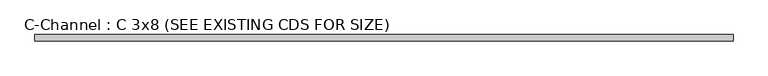
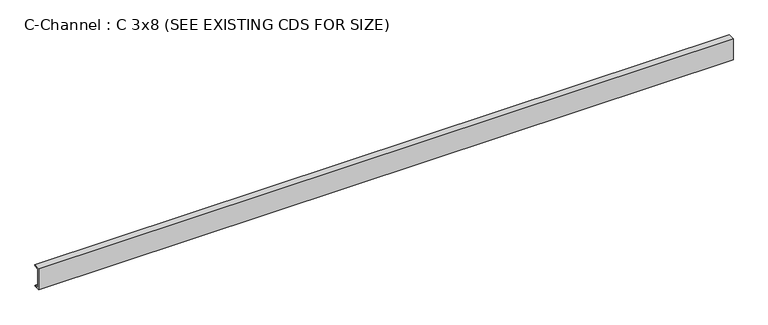
"""IFC4 building model written with IfcOpenShell, lengths in millimetres: beam geometry, C-Channel : C 3x8 (SEE EXISTING CDS FOR SIZE)."""

import ifcopenshell
import ifcopenshell.guid

model = None  # the IFC model being written
_history = None  # IfcOwnerHistory: only IFC2X3 demands one
_inside = {}  # id of a spatial element -> (the spatial element, [elements in it])
_under = {}  # id of a project, library or spatial element -> (it, [spatial elements below it])
_declared = {}  # id of a project -> (the project, [libraries it declares])
_typed = {}  # id of a type object -> (the type object, [elements of that type])
_made_of = {}  # id of a material, layer set ... -> (it, [elements and type objects made of it])


def new_model(schema):
    """Start an empty IFC model of exactly this schema.

    Asked for "IFC4X3", IfcOpenShell would pick the latest addendum, in which some entities
    have other attributes; the version numbers below select the first issue.
    IFC2X3 requires an IfcOwnerHistory on every rooted entity: one is made here for all.
    """
    global model, _history
    if schema == "IFC4X3":
        model = ifcopenshell.file(schema_version=(4, 3, 0, 0))
    else:
        model = ifcopenshell.file(schema=schema)
    _inside.clear()
    _under.clear()
    _declared.clear()
    _typed.clear()
    _made_of.clear()
    _history = None
    if model.schema == "IFC2X3":
        org = make("IfcOrganization", Name="unknown")
        user = make(
            "IfcPersonAndOrganization",
            ThePerson=make("IfcPerson", FamilyName="unknown"),
            TheOrganization=org,
        )
        app = make(
            "IfcApplication",
            ApplicationDeveloper=org,
            Version="unknown",
            ApplicationFullName="unknown",
            ApplicationIdentifier="unknown",
        )
        _history = make(
            "IfcOwnerHistory",
            OwningUser=user,
            OwningApplication=app,
            ChangeAction="ADDED",
            CreationDate=0,
        )
    return model


def make(cls, **values):
    """One entity of the class cls with the attributes given. An attribute that is None is left unset."""
    return model.create_entity(
        cls, **{name: value for name, value in values.items() if value is not None}
    )


def rooted(cls, **values):
    """An entity with a GlobalId (a new one), such as an element, a storey or a relation."""
    return make(cls, GlobalId=ifcopenshell.guid.new(), OwnerHistory=_history, **values)


def si_unit(unit_type, name, prefix=None):
    """IfcSIUnit, for example si_unit("LENGTHUNIT", "METRE", prefix="MILLI")."""
    return make("IfcSIUnit", UnitType=unit_type, Prefix=prefix, Name=name)


def assignment(units):
    """IfcUnitAssignment: the units of a project."""
    return None if units is None else make("IfcUnitAssignment", Units=units)


def point(xyz):
    """IfcCartesianPoint."""
    return None if xyz is None else make("IfcCartesianPoint", Coordinates=xyz)


def direction(xyz):
    """IfcDirection."""
    return None if xyz is None else make("IfcDirection", DirectionRatios=xyz)


def frame(location, z_axis=None, x_axis=None):
    """IfcAxis2Placement3D, a coordinate frame: its origin and axes. An axis left out is left unset."""
    return make(
        "IfcAxis2Placement3D",
        Location=point(location),
        Axis=direction(z_axis),
        RefDirection=direction(x_axis),
    )


def frame_2d(location, x_axis=None):
    """IfcAxis2Placement2D, a coordinate frame in the plane: its origin and x axis."""
    return make(
        "IfcAxis2Placement2D", Location=point(location), RefDirection=direction(x_axis)
    )


def origin():
    """The frame at (0, 0, 0) with its axes left unset."""
    return frame((0.0, 0.0, 0.0))


def place(relative_to, where):
    """IfcLocalPlacement: puts the frame where relative to a parent placement (None: the world)."""
    return make(
        "IfcLocalPlacement", PlacementRelTo=relative_to, RelativePlacement=where
    )


def context(
    kind, dimensions, precision=None, world=None, true_north=None, identifier=None
):
    """IfcGeometricRepresentationContext, for example the 3D "Model" context."""
    return make(
        "IfcGeometricRepresentationContext",
        ContextIdentifier=identifier,
        ContextType=kind,
        CoordinateSpaceDimension=dimensions,
        Precision=precision,
        WorldCoordinateSystem=world,
        TrueNorth=true_north,
    )


def project(units=None, contexts=None):
    """IfcProject with its units and contexts."""
    return rooted(
        "IfcProject",
        Name="project",
        RepresentationContexts=contexts,
        UnitsInContext=assignment(units),
    )


def spatial(cls, under=None, at=None, **own):
    """A site, building, storey or space (cls), placed at a placement, below another one or the project."""
    s = rooted(cls, ObjectPlacement=at, **own)
    if under is not None:
        _under.setdefault(under.id(), (under, []))[1].append(s)
    return s


def polyline(points):
    """IfcPolyline through the points."""
    return make("IfcPolyline", Points=[point(p) for p in points])


def circle_curve(where, radius):
    """IfcCircle in the frame where."""
    return make("IfcCircle", Position=where, Radius=radius)


def trimmed(basis, trim1, trim2, sense, master):
    """IfcTrimmedCurve: the piece of a basis curve between two trims."""
    return make(
        "IfcTrimmedCurve",
        BasisCurve=basis,
        Trim1=trim1,
        Trim2=trim2,
        SenseAgreement=sense,
        MasterRepresentation=master,
    )


def segment(curve, same_sense, transition):
    """IfcCompositeCurveSegment."""
    return make(
        "IfcCompositeCurveSegment",
        Transition=transition,
        SameSense=same_sense,
        ParentCurve=curve,
    )


def composite_curve(segments, self_intersect=None):
    """IfcCompositeCurve: segments joined end to end."""
    return make("IfcCompositeCurve", Segments=segments, SelfIntersect=self_intersect)


def outline(outer, holes=None, kind="AREA"):
    """IfcArbitraryClosedProfileDef: a profile drawn as a closed curve; with holes, ...WithVoids."""
    if holes is None:
        return make("IfcArbitraryClosedProfileDef", ProfileType=kind, OuterCurve=outer)
    return make(
        "IfcArbitraryProfileDefWithVoids",
        ProfileType=kind,
        OuterCurve=outer,
        InnerCurves=holes,
    )


def extrude(swept, where, along, depth):
    """IfcExtrudedAreaSolid: the profile swept, set in the frame where, extruded along a direction by depth."""
    return make(
        "IfcExtrudedAreaSolid",
        SweptArea=swept,
        Position=where,
        ExtrudedDirection=direction(along),
        Depth=depth,
    )


def shape(context_of_items, identifier, shape_type, items):
    """IfcShapeRepresentation: the items that make up one representation, for example the "Body"."""
    return make(
        "IfcShapeRepresentation",
        ContextOfItems=context_of_items,
        RepresentationIdentifier=identifier,
        RepresentationType=shape_type,
        Items=items,
    )


def source(mapping_origin, context_of_items, identifier, shape_type, items):
    """IfcRepresentationMap: a shape defined once, which mapped items show again and again."""
    return make(
        "IfcRepresentationMap",
        MappingOrigin=mapping_origin,
        MappedRepresentation=shape(context_of_items, identifier, shape_type, items),
    )


def transform(
    local_origin,
    x_axis=None,
    y_axis=None,
    z_axis=None,
    scale=None,
    scale2=None,
    scale3=None,
    uniform=True,
):
    """IfcCartesianTransformationOperator3D, or its non-uniform kind. x_axis, y_axis, z_axis: its Axis1, 2, 3."""
    if uniform:
        return make(
            "IfcCartesianTransformationOperator3D",
            Axis1=direction(x_axis),
            Axis2=direction(y_axis),
            LocalOrigin=point(local_origin),
            Scale=scale,
            Axis3=direction(z_axis),
        )
    return make(
        "IfcCartesianTransformationOperator3DnonUniform",
        Axis1=direction(x_axis),
        Axis2=direction(y_axis),
        LocalOrigin=point(local_origin),
        Scale=scale,
        Axis3=direction(z_axis),
        Scale2=scale2,
        Scale3=scale3,
    )


def mapped(mapping_source, mapping_target):
    """IfcMappedItem: shows the shape of a source again, moved by a transform."""
    return make(
        "IfcMappedItem", MappingSource=mapping_source, MappingTarget=mapping_target
    )


def made_of(thing, what):
    """Note that an element or type object is made of a material, layer set ...; save() writes the relation."""
    if what is not None:
        _made_of.setdefault(what.id(), (what, []))[1].append(thing)
    return thing


def element(
    cls,
    number,
    at=None,
    inside=None,
    cuts=None,
    type_object=None,
    material=None,
    context=None,
    identifier="Body",
    shape_type=None,
    held_by="IfcProductDefinitionShape",
    body=None,
    shapes=None,
    **own,
):
    """One element of the class cls, such as IfcWall. Its Tag is "e" and its number.

    at: its placement. inside: the storey or other place that contains it. cuts: it is an
    opening in that element (IfcRelVoidsElement). A single representation is given by context,
    identifier, shape_type and body (its items); several are given by shapes. held_by: the class
    of the entity that holds the representations. save() writes the other relations.
    """
    e = rooted(cls, Tag="e%d" % number, ObjectPlacement=at, **own)
    if body is not None:
        shapes = [shape(context, identifier, shape_type, body)]
    if shapes is not None:
        e.Representation = make(held_by, Representations=shapes)
    if inside is not None:
        _inside.setdefault(inside.id(), (inside, []))[1].append(e)
    if cuts is not None:
        rooted(
            "IfcRelVoidsElement", RelatingBuildingElement=cuts, RelatedOpeningElement=e
        )
    if type_object is not None:
        _typed.setdefault(type_object.id(), (type_object, []))[1].append(e)
    return made_of(e, material)


def aggregate(whole, parts):
    """IfcRelAggregates: a whole, such as a stair, and the parts it consists of."""
    return rooted("IfcRelAggregates", RelatingObject=whole, RelatedObjects=parts)


def save(model, path):
    """Write the relations noted so far, then the file.

    IfcRelAggregates (storeys below a building ...), IfcRelContainedInSpatialStructure (elements
    in a storey), IfcRelDefinesByType, IfcRelAssociatesMaterial and IfcRelDeclares: one each for
    every whole, place, type object, material and project.
    """
    for whole, parts in _under.values():
        aggregate(whole, parts)
    for where, things in _inside.values():
        rooted(
            "IfcRelContainedInSpatialStructure",
            RelatedElements=things,
            RelatingStructure=where,
        )
    for kind, things in _typed.values():
        rooted("IfcRelDefinesByType", RelatedObjects=things, RelatingType=kind)
    for what, things in _made_of.values():
        rooted("IfcRelAssociatesMaterial", RelatedObjects=things, RelatingMaterial=what)
    for by, libraries in _declared.values():
        rooted("IfcRelDeclares", RelatingContext=by, RelatedDefinitions=libraries)
    model.write(path)


def c_channel_c_3x8_see_existing_cds_for_size_48e3e816(model_context):
    return source(origin(), model_context, "Body", "SweptSolid", [
        extrude(outline(composite_curve([segment(polyline([(-13.5128, 101.6), (44.9072, 101.6)]), True, "CONTINUOUS"), segment(trimmed(circle_curve(frame_2d((35.6108, 101.6)), 9.2964), [point((44.9072, 101.6))], [point((35.6108, 92.3036))], False, "CARTESIAN"), True, "CONTINUOUS"), segment(polyline([(35.6108, 92.3036), (-2.8702, 86.2088084), (-2.8702, -86.2088084), (35.6108, -92.3036)]), True, "CONTINUOUS"), segment(trimmed(circle_curve(frame_2d((35.6108, -101.6)), 9.2964), [point((35.6108, -92.3036))], [point((44.9072, -101.6))], False, "CARTESIAN"), True, "CONTINUOUS"), segment(polyline([(44.9072, -101.6), (-13.5128, -101.6), (-13.5128, 101.6)]), True, "CONTINUOUS")], self_intersect=False)), frame((-3168.6499994, 0.0, 0.0), z_axis=(1.0, 0.0, 0.0), x_axis=(0.0, 1.0, 0.0)), (0.0, 0.0, 1.0), 6337.2999994),
    ])


if __name__ == "__main__":
    model = new_model("IFC4")
    model_context = context("Model", 3, world=origin())
    ifc_project = project(units=[si_unit("LENGTHUNIT", "METRE", prefix="MILLI")], contexts=[model_context])
    site = spatial("IfcSite", under=ifc_project)
    building = spatial("IfcBuilding", under=site)
    placement = place(None, origin())
    c_channel_c_3x8_see_existing_cds_for_size_shape = c_channel_c_3x8_see_existing_cds_for_size_48e3e816(model_context)
    element("IfcBeam", 1, ObjectType="C-Channel : C 3x8 (SEE EXISTING CDS FOR SIZE)", at=placement, inside=building, context=model_context, shape_type="MappedRepresentation", body=[
        mapped(c_channel_c_3x8_see_existing_cds_for_size_shape, transform((0.0, 0.0, 0.0), x_axis=(1.0, 0.0, 0.0), y_axis=(0.0, 1.0, 0.0), z_axis=(0.0, 0.0, 1.0))),
    ])
    save(model, "model.ifc")

# Revit data of these elements
# Type "C-Channel : C 3x8 (SEE EXISTING CDS FOR SIZE)"
#   Assembly Code = "B10"
#   W = 14.7
#   Length [instance default] = 5' - 0"
#   bf = 0' - 2.3"
#   d = 0' - 8"
#   tf = 0' - 0.366"
#   tw = 0' - 0.419"
#   x = 0' - 0.532"
#   A = 0.0300694 SF
#   Structural Material [instance default] = Steel ASTM A36
# Element 1 (IfcBeam, "C-Channel : C 3x8 (SEE EXISTING CDS FOR SIZE)")
#   Materials on its faces: "Steel ASTM A36"
# Materials
#   "Steel ASTM A36": class "Metal", colour RGB 199 199 199, transparency 0, Description = "Structural steel, ASTM A36 Grade B, mill finish", Cost = 0
